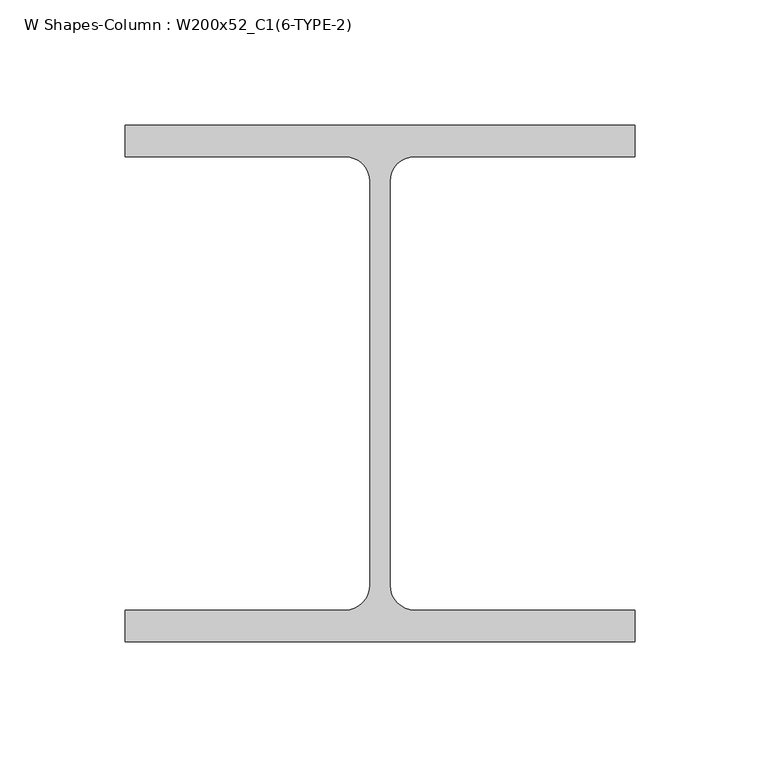
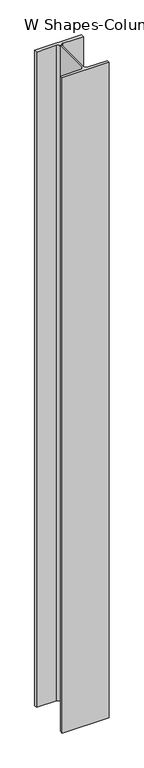
"""IFC4 building model written with IfcOpenShell, lengths in millimetres: column geometry, W Shapes-Column : W200x52_C1(6-TYPE-2)."""

import ifcopenshell
import ifcopenshell.guid

model = None  # the IFC model being written
_history = None  # IfcOwnerHistory: only IFC2X3 demands one
_inside = {}  # id of a spatial element -> (the spatial element, [elements in it])
_under = {}  # id of a project, library or spatial element -> (it, [spatial elements below it])
_declared = {}  # id of a project -> (the project, [libraries it declares])
_typed = {}  # id of a type object -> (the type object, [elements of that type])
_made_of = {}  # id of a material, layer set ... -> (it, [elements and type objects made of it])


def new_model(schema):
    """Start an empty IFC model of exactly this schema.

    Asked for "IFC4X3", IfcOpenShell would pick the latest addendum, in which some entities
    have other attributes; the version numbers below select the first issue.
    IFC2X3 requires an IfcOwnerHistory on every rooted entity: one is made here for all.
    """
    global model, _history
    if schema == "IFC4X3":
        model = ifcopenshell.file(schema_version=(4, 3, 0, 0))
    else:
        model = ifcopenshell.file(schema=schema)
    _inside.clear()
    _under.clear()
    _declared.clear()
    _typed.clear()
    _made_of.clear()
    _history = None
    if model.schema == "IFC2X3":
        org = make("IfcOrganization", Name="unknown")
        user = make(
            "IfcPersonAndOrganization",
            ThePerson=make("IfcPerson", FamilyName="unknown"),
            TheOrganization=org,
        )
        app = make(
            "IfcApplication",
            ApplicationDeveloper=org,
            Version="unknown",
            ApplicationFullName="unknown",
            ApplicationIdentifier="unknown",
        )
        _history = make(
            "IfcOwnerHistory",
            OwningUser=user,
            OwningApplication=app,
            ChangeAction="ADDED",
            CreationDate=0,
        )
    return model


def make(cls, **values):
    """One entity of the class cls with the attributes given. An attribute that is None is left unset."""
    return model.create_entity(
        cls, **{name: value for name, value in values.items() if value is not None}
    )


def rooted(cls, **values):
    """An entity with a GlobalId (a new one), such as an element, a storey or a relation."""
    return make(cls, GlobalId=ifcopenshell.guid.new(), OwnerHistory=_history, **values)


def si_unit(unit_type, name, prefix=None):
    """IfcSIUnit, for example si_unit("LENGTHUNIT", "METRE", prefix="MILLI")."""
    return make("IfcSIUnit", UnitType=unit_type, Prefix=prefix, Name=name)


def assignment(units):
    """IfcUnitAssignment: the units of a project."""
    return None if units is None else make("IfcUnitAssignment", Units=units)


def point(xyz):
    """IfcCartesianPoint."""
    return None if xyz is None else make("IfcCartesianPoint", Coordinates=xyz)


def direction(xyz):
    """IfcDirection."""
    return None if xyz is None else make("IfcDirection", DirectionRatios=xyz)


def frame(location, z_axis=None, x_axis=None):
    """IfcAxis2Placement3D, a coordinate frame: its origin and axes. An axis left out is left unset."""
    return make(
        "IfcAxis2Placement3D",
        Location=point(location),
        Axis=direction(z_axis),
        RefDirection=direction(x_axis),
    )


def frame_2d(location, x_axis=None):
    """IfcAxis2Placement2D, a coordinate frame in the plane: its origin and x axis."""
    return make(
        "IfcAxis2Placement2D", Location=point(location), RefDirection=direction(x_axis)
    )


def origin():
    """The frame at (0, 0, 0) with its axes left unset."""
    return frame((0.0, 0.0, 0.0))


def place(relative_to, where):
    """IfcLocalPlacement: puts the frame where relative to a parent placement (None: the world)."""
    return make(
        "IfcLocalPlacement", PlacementRelTo=relative_to, RelativePlacement=where
    )


def context(
    kind, dimensions, precision=None, world=None, true_north=None, identifier=None
):
    """IfcGeometricRepresentationContext, for example the 3D "Model" context."""
    return make(
        "IfcGeometricRepresentationContext",
        ContextIdentifier=identifier,
        ContextType=kind,
        CoordinateSpaceDimension=dimensions,
        Precision=precision,
        WorldCoordinateSystem=world,
        TrueNorth=true_north,
    )


def project(units=None, contexts=None):
    """IfcProject with its units and contexts."""
    return rooted(
        "IfcProject",
        Name="project",
        RepresentationContexts=contexts,
        UnitsInContext=assignment(units),
    )


def spatial(cls, under=None, at=None, **own):
    """A site, building, storey or space (cls), placed at a placement, below another one or the project."""
    s = rooted(cls, ObjectPlacement=at, **own)
    if under is not None:
        _under.setdefault(under.id(), (under, []))[1].append(s)
    return s


def polyline(points):
    """IfcPolyline through the points."""
    return make("IfcPolyline", Points=[point(p) for p in points])


def circle_curve(where, radius):
    """IfcCircle in the frame where."""
    return make("IfcCircle", Position=where, Radius=radius)


def trimmed(basis, trim1, trim2, sense, master):
    """IfcTrimmedCurve: the piece of a basis curve between two trims."""
    return make(
        "IfcTrimmedCurve",
        BasisCurve=basis,
        Trim1=trim1,
        Trim2=trim2,
        SenseAgreement=sense,
        MasterRepresentation=master,
    )


def segment(curve, same_sense, transition):
    """IfcCompositeCurveSegment."""
    return make(
        "IfcCompositeCurveSegment",
        Transition=transition,
        SameSense=same_sense,
        ParentCurve=curve,
    )


def composite_curve(segments, self_intersect=None):
    """IfcCompositeCurve: segments joined end to end."""
    return make("IfcCompositeCurve", Segments=segments, SelfIntersect=self_intersect)


def outline(outer, holes=None, kind="AREA"):
    """IfcArbitraryClosedProfileDef: a profile drawn as a closed curve; with holes, ...WithVoids."""
    if holes is None:
        return make("IfcArbitraryClosedProfileDef", ProfileType=kind, OuterCurve=outer)
    return make(
        "IfcArbitraryProfileDefWithVoids",
        ProfileType=kind,
        OuterCurve=outer,
        InnerCurves=holes,
    )


def extrude(swept, where, along, depth):
    """IfcExtrudedAreaSolid: the profile swept, set in the frame where, extruded along a direction by depth."""
    return make(
        "IfcExtrudedAreaSolid",
        SweptArea=swept,
        Position=where,
        ExtrudedDirection=direction(along),
        Depth=depth,
    )


def shape(context_of_items, identifier, shape_type, items):
    """IfcShapeRepresentation: the items that make up one representation, for example the "Body"."""
    return make(
        "IfcShapeRepresentation",
        ContextOfItems=context_of_items,
        RepresentationIdentifier=identifier,
        RepresentationType=shape_type,
        Items=items,
    )


def source(mapping_origin, context_of_items, identifier, shape_type, items):
    """IfcRepresentationMap: a shape defined once, which mapped items show again and again."""
    return make(
        "IfcRepresentationMap",
        MappingOrigin=mapping_origin,
        MappedRepresentation=shape(context_of_items, identifier, shape_type, items),
    )


def transform(
    local_origin,
    x_axis=None,
    y_axis=None,
    z_axis=None,
    scale=None,
    scale2=None,
    scale3=None,
    uniform=True,
):
    """IfcCartesianTransformationOperator3D, or its non-uniform kind. x_axis, y_axis, z_axis: its Axis1, 2, 3."""
    if uniform:
        return make(
            "IfcCartesianTransformationOperator3D",
            Axis1=direction(x_axis),
            Axis2=direction(y_axis),
            LocalOrigin=point(local_origin),
            Scale=scale,
            Axis3=direction(z_axis),
        )
    return make(
        "IfcCartesianTransformationOperator3DnonUniform",
        Axis1=direction(x_axis),
        Axis2=direction(y_axis),
        LocalOrigin=point(local_origin),
        Scale=scale,
        Axis3=direction(z_axis),
        Scale2=scale2,
        Scale3=scale3,
    )


def mapped(mapping_source, mapping_target):
    """IfcMappedItem: shows the shape of a source again, moved by a transform."""
    return make(
        "IfcMappedItem", MappingSource=mapping_source, MappingTarget=mapping_target
    )


def made_of(thing, what):
    """Note that an element or type object is made of a material, layer set ...; save() writes the relation."""
    if what is not None:
        _made_of.setdefault(what.id(), (what, []))[1].append(thing)
    return thing


def element(
    cls,
    number,
    at=None,
    inside=None,
    cuts=None,
    type_object=None,
    material=None,
    context=None,
    identifier="Body",
    shape_type=None,
    held_by="IfcProductDefinitionShape",
    body=None,
    shapes=None,
    **own,
):
    """One element of the class cls, such as IfcWall. Its Tag is "e" and its number.

    at: its placement. inside: the storey or other place that contains it. cuts: it is an
    opening in that element (IfcRelVoidsElement). A single representation is given by context,
    identifier, shape_type and body (its items); several are given by shapes. held_by: the class
    of the entity that holds the representations. save() writes the other relations.
    """
    e = rooted(cls, Tag="e%d" % number, ObjectPlacement=at, **own)
    if body is not None:
        shapes = [shape(context, identifier, shape_type, body)]
    if shapes is not None:
        e.Representation = make(held_by, Representations=shapes)
    if inside is not None:
        _inside.setdefault(inside.id(), (inside, []))[1].append(e)
    if cuts is not None:
        rooted(
            "IfcRelVoidsElement", RelatingBuildingElement=cuts, RelatedOpeningElement=e
        )
    if type_object is not None:
        _typed.setdefault(type_object.id(), (type_object, []))[1].append(e)
    return made_of(e, material)


def aggregate(whole, parts):
    """IfcRelAggregates: a whole, such as a stair, and the parts it consists of."""
    return rooted("IfcRelAggregates", RelatingObject=whole, RelatedObjects=parts)


def save(model, path):
    """Write the relations noted so far, then the file.

    IfcRelAggregates (storeys below a building ...), IfcRelContainedInSpatialStructure (elements
    in a storey), IfcRelDefinesByType, IfcRelAssociatesMaterial and IfcRelDeclares: one each for
    every whole, place, type object, material and project.
    """
    for whole, parts in _under.values():
        aggregate(whole, parts)
    for where, things in _inside.values():
        rooted(
            "IfcRelContainedInSpatialStructure",
            RelatedElements=things,
            RelatingStructure=where,
        )
    for kind, things in _typed.values():
        rooted("IfcRelDefinesByType", RelatedObjects=things, RelatingType=kind)
    for what, things in _made_of.values():
        rooted("IfcRelAssociatesMaterial", RelatedObjects=things, RelatingMaterial=what)
    for by, libraries in _declared.values():
        rooted("IfcRelDeclares", RelatingContext=by, RelatedDefinitions=libraries)
    model.write(path)


def w_shapes_column_w200x52_c1_6_type_2_d7336851(model_context):
    return source(origin(), model_context, "Body", "SweptSolid", [
        extrude(outline(composite_curve([segment(polyline([(101.854, 103.124), (101.854, 90.551), (13.9446, 90.551)]), True, "CONTINUOUS"), segment(trimmed(circle_curve(frame_2d((13.9446, 80.5434)), 10.0076), [point((13.9446, 90.551))], [point((3.937, 80.5434))], True, "CARTESIAN"), True, "CONTINUOUS"), segment(polyline([(3.937, 80.5434), (3.937, -80.5434)]), True, "CONTINUOUS"), segment(trimmed(circle_curve(frame_2d((13.9446, -80.5434)), 10.0076), [point((3.937, -80.5434))], [point((13.9446, -90.551))], True, "CARTESIAN"), True, "CONTINUOUS"), segment(polyline([(13.9446, -90.551), (101.854, -90.551), (101.854, -103.124), (-101.854, -103.124), (-101.854, -90.551), (-13.9446, -90.551)]), True, "CONTINUOUS"), segment(trimmed(circle_curve(frame_2d((-13.9446, -80.5434)), 10.0076), [point((-13.9446, -90.551))], [point((-3.937, -80.5434))], True, "CARTESIAN"), True, "CONTINUOUS"), segment(polyline([(-3.937, -80.5434), (-3.937, 80.5434)]), True, "CONTINUOUS"), segment(trimmed(circle_curve(frame_2d((-13.9446, 80.5434)), 10.0076), [point((-3.937, 80.5434))], [point((-13.9446, 90.551))], True, "CARTESIAN"), True, "CONTINUOUS"), segment(polyline([(-13.9446, 90.551), (-101.854, 90.551), (-101.854, 103.124), (101.854, 103.124)]), True, "CONTINUOUS")], self_intersect=False)), frame((0.0, 0.0, 9260.0), z_axis=(0.0, 0.0, 1.0), x_axis=(1.0, 0.0, 0.0)), (0.0, 0.0, 1.0), 3000.0),
    ])


if __name__ == "__main__":
    model = new_model("IFC4")
    model_context = context("Model", 3, world=origin())
    ifc_project = project(units=[si_unit("LENGTHUNIT", "METRE", prefix="MILLI")], contexts=[model_context])
    site = spatial("IfcSite", under=ifc_project)
    building = spatial("IfcBuilding", under=site)
    placement = place(None, origin())
    w_shapes_column_w200x52_c1_6_type_2_shape = w_shapes_column_w200x52_c1_6_type_2_d7336851(model_context)
    element("IfcColumn", 1, ObjectType="W Shapes-Column : W200x52_C1(6-TYPE-2)", at=placement, inside=building, context=model_context, shape_type="MappedRepresentation", body=[
        mapped(w_shapes_column_w200x52_c1_6_type_2_shape, transform((0.0, 0.0, 0.0), x_axis=(1.0, 0.0, 0.0), y_axis=(0.0, 1.0, 0.0), z_axis=(0.0, 0.0, 1.0))),
    ])
    save(model, "model.ifc")

# Revit data of these elements
# Type "W Shapes-Column : W200x52_C1(6-TYPE-2)"
#   Section Name Key = "W8X35"
#   Assembly Code = "B10"
#   Width = 20.3708 cm
#   Web Thickness = 0.7874 cm
#   Web Fillet = 1.0008 cm
#   Warping Constant = 166223.7 cm⁶
#   Torsional Moment of Inertia = 32.0082 cm⁴
#   Section Area = 66.4515 cm²
#   Plastic Modulus weak axis = 263.832 cm³
#   Plastic Modulus strong axis = 568.631 cm³
#   Perimeter = 1.1936 m²/m
#   Nominal Weight = 52.0857 kgf/m
#   Moment of Inertia weak axis = 1773.15 cm⁴
#   Moment of Inertia strong axis = 5286.14 cm⁴
#   Height = 20.6248 cm
#   Flange Thickness = 1.2573 cm
#   Elastic Modulus weak axis = 173.703 cm³
#   Elastic Modulus strong axis = 511.276 cm³
#   Clear Web Height = 14.605 cm
#   Centroid Vertical = 10.3124 cm
#   Centroid Horizontal = 10.1854 cm
#   Bolt Spacing = 13.97 cm
#   Structural Material [instance default] = Steel ASTM A992
#   Principal Axes Angle = 0
# Element 1 (IfcColumn, "W Shapes-Column : W200x52_C1(6-TYPE-2)")
#   Structural Material = none
# Materials
#   "Steel ASTM A992": class "Metal", colour RGB 199 199 199, transparency 0, Description = "Structural steel 50ksi", Cost = 0
